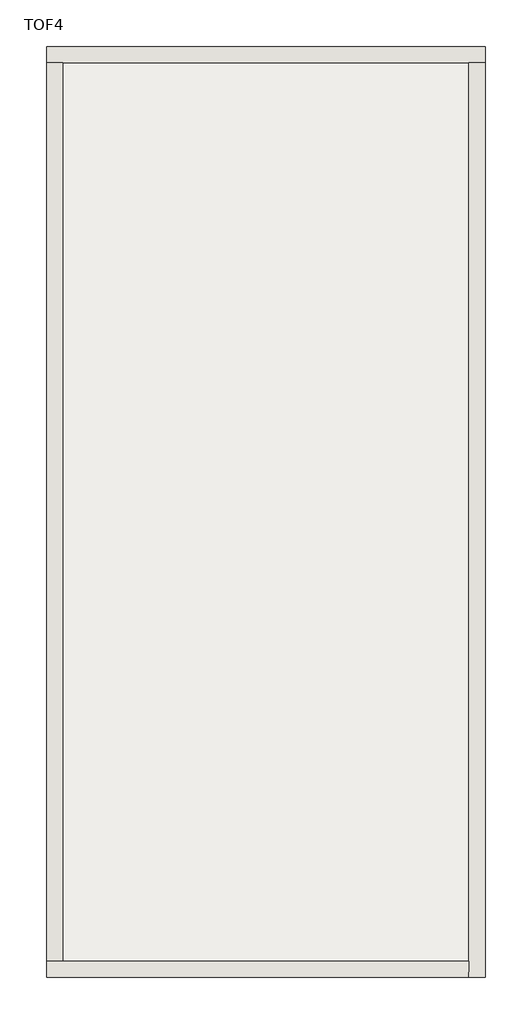
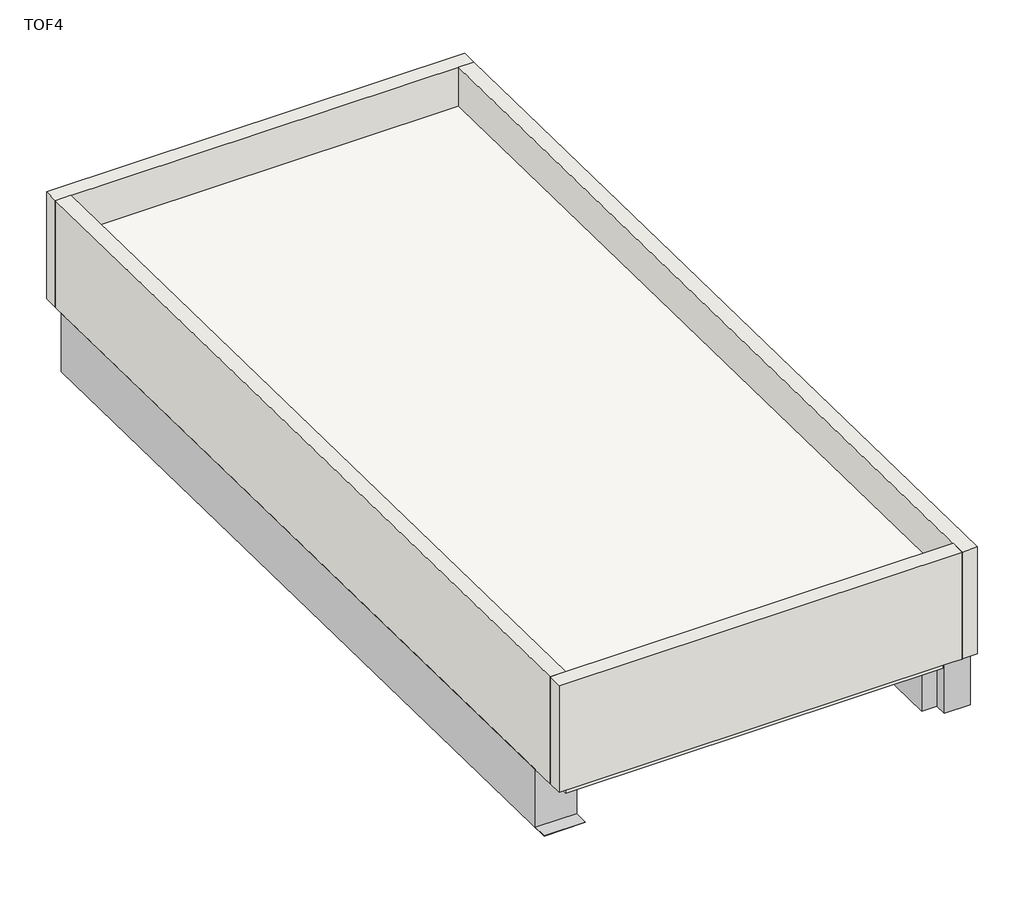
# One storey: 4 walls, 2 beams, 2 slabs.
"""IFC4 building model written with IfcOpenShell, lengths in millimetres."""

from ifc_helpers import new_model, si_unit, frame, origin, place, context, project, spatial, polyline, outline, extrude, faceted_brep, element, save

model = new_model("IFC4")

# Units and contexts
model_context = context("Model", 3, world=origin())
ifc_project = project(units=[si_unit("LENGTHUNIT", "METRE", prefix="MILLI")], contexts=[model_context])

# Site, building, storey
site = spatial("IfcSite", under=ifc_project)
building = spatial("IfcBuilding", under=site)
storey = spatial("IfcBuildingStorey", under=building, Name="TOF4", Elevation=19209.9618634)

# Beams
placement = place(None, origin())
element("IfcBeam", 1, ObjectType="RC Beam_Rectangular : H_SB_AR_S16_AG_B400xH600_PHWG1", at=placement, inside=storey, context=model_context, shape_type="Brep", body=[
    faceted_brep([(50825.0, 9549.5208589, 19206.0830755), (51225.0, 9549.5208589, 19206.0830755), (51225.0, 17599.5208589, 19049.9618634), (50825.0, 17599.5208589, 19049.9618634), (50825.0, 9549.5208589, 18609.9618634), (50825.0, 17549.5208589, 19049.9618634), (50825.0, 17549.5208589, 18450.8187335), (50825.0, 9399.5208589, 18608.8793395), (50825.0, 9399.5208589, 18609.9618634), (51225.0, 17549.5208589, 18450.8187335), (51225.0, 9399.5208589, 18608.8793395), (51225.0, 9549.5208589, 18609.9618634), (51225.0, 9399.5208589, 18609.9618634), (51225.0, 17549.5208589, 19049.9618634), (51075.0, 9549.5208589, 18609.9618634)], [[[0, 1, 2, 3]], [[4, 0, 3, 5, 6, 7, 8]], [[6, 9, 10, 7]], [[1, 11, 12, 10, 9, 13, 2]], [[11, 14, 4, 8, 12]], [[4, 14, 11, 1, 0]], [[5, 13, 9, 6]], [[13, 5, 3, 2]], [[8, 7, 10, 12]]]),
])
element("IfcBeam", 2, ObjectType="RC Beam_Rectangular : H_SB_AR_S16_AG_B400xH600_PHWG1", at=placement, inside=storey, context=model_context, shape_type="Brep", body=[
    faceted_brep([(54900.0, 9274.5208589, 19211.4164088), (54900.0, 17599.5208589, 19049.9618634), (54500.0, 17599.5208589, 19049.9618634), (54500.0, 9549.5208589, 19206.0830755), (54500.0, 9399.5208589, 19208.9921664), (54750.0, 9399.5208589, 19208.9921664), (54750.0, 9349.5208589, 19209.9618634), (54500.0, 9349.5208589, 19209.9618634), (54500.0, 9299.5208589, 19210.9315603), (54750.0, 9299.5208589, 19210.9315603), (54750.0, 9274.5208589, 19211.4164088), (54500.0, 9299.5208589, 19209.9618634), (54900.0, 17549.5208589, 18450.8187335), (54900.0, 9274.5208589, 18611.303582), (54650.0, 9274.5208589, 18611.303582), (54650.0, 9399.5208589, 18608.8793395), (54500.0, 9399.5208589, 18608.8793395), (54500.0, 17549.5208589, 18450.8187335), (54900.0, 17549.5208589, 19049.9618634), (54500.0, 17549.5208589, 19049.9618634), (54750.0, 9274.5208589, 19206.6647429), (54650.0, 9274.5208589, 19206.6647429), (54650.0, 9399.5208589, 19206.6647429), (54750.0, 9399.5208589, 19206.6647429), (54750.0, 9299.5208589, 19209.9618634)], [[[0, 1, 2, 3, 4, 5, 6, 7, 8, 9, 10]], [[8, 7, 11]], [[12, 13, 14, 15, 16, 17]], [[1, 0, 13, 12, 18]], [[19, 18, 12, 17]], [[18, 19, 2, 1]], [[13, 0, 10, 20, 21, 14]], [[22, 23, 5, 4, 16, 15]], [[7, 6, 24, 11]], [[23, 22, 21, 20]], [[22, 15, 14, 21]], [[5, 23, 20, 10, 9, 24, 6]], [[24, 9, 8, 11]], [[19, 17, 16, 4, 3, 2]]]),
])

# Slabs
element("IfcSlab", 3, ObjectType="H_FL_AR_S17_RC Slab T150_PHRS1", at=placement, inside=storey, context=model_context, shape_type="SweptSolid", body=[
    extrude(outline(polyline([(17649.5208589, 18899.9343282), (9299.5208589, 19059.9343282), (9299.5208589, 19209.9618634), (17649.5208589, 19049.9618634), (17649.5208589, 18899.9343282)])), frame((50975.0, 0.0, 0.0), z_axis=(1.0, 0.0, 0.0), x_axis=(0.0, 1.0, 0.0)), (0.0, 0.0, 1.0), 3775.0),
])
element("IfcSlab", 4, ObjectType="H_RF_AR_B06_Roof Finish", at=placement, inside=storey, context=model_context, shape_type="SweptSolid", body=[
    extrude(outline(polyline([(17649.5208589, 19399.8976154), (9299.4677289, 19559.8976154), (9299.4677289, 19909.9618634), (17649.5208589, 19749.9618634), (17649.5208589, 19399.8976154)])), frame((50975.0, 0.0, 0.0), z_axis=(1.0, 0.0, 0.0), x_axis=(0.0, 1.0, 0.0)), (0.0, 0.0, 1.0), 3775.0),
])

# Walls
element("IfcWall", 5, ObjectType="H_WA_AR_B02_Ext Wall_RC T150_parapet", at=placement, inside=storey, context=model_context, shape_type="SweptSolid", body=[
    extrude(outline(polyline([(19049.9618634, 51075.0), (19049.9618634, 54650.0), (19051.3766309, 54650.0), (19051.3766309, 54900.0), (20149.9618634, 54900.0), (20149.9618634, 50825.0), (19051.3766309, 50825.0), (19051.3766309, 51075.0), (19049.9618634, 51075.0)])), frame((0.0, 17649.5208589, 0.0), z_axis=(0.0, 1.0, 0.0), x_axis=(0.0, 0.0, 1.0)), (0.0, 0.0, 1.0), 150.0),
])
element("IfcWall", 6, ObjectType="H_WA_AR_B02_Ext Wall_RC T150_parapet", at=placement, inside=storey, context=model_context, shape_type="Brep", body=[
    faceted_brep([(54750.0, 17649.5208589, 20151.3736281), (54750.0, 17649.5208589, 19051.3736281), (54750.0, 9149.5208589, 19211.3736281), (54750.0, 9149.5208589, 20309.9618634), (54750.0, 9149.5208589, 20311.3736281), (54900.0, 17649.5208589, 19051.3736281), (54900.0, 17649.5208589, 20149.9618634), (54900.0, 17649.5208589, 20151.3736281), (54900.0, 9149.5208589, 20311.3736281), (54900.0, 9149.5208589, 19211.3736281), (54900.0, 17549.5208589, 19053.255981)], [[[0, 1, 2, 3, 4]], [[5, 6, 7, 8, 9, 10]], [[4, 3, 2, 9, 8]], [[2, 1, 5, 10, 9]], [[0, 4, 8, 7]], [[0, 7, 6, 5, 1]]]),
])
element("IfcWall", 7, ObjectType="H_WA_AR_B02_Ext Wall_RC T150_parapet", at=placement, inside=storey, context=model_context, shape_type="Brep", body=[
    faceted_brep([(54750.0, 9299.5208589, 19209.9618634), (54500.0, 9299.5208589, 19209.9618634), (50975.0, 9299.5208589, 19209.9618634), (50825.0, 9299.5208589, 19209.9618634), (50825.0, 9299.5208589, 20308.5500987), (50825.0, 9299.5208589, 20309.9618634), (54750.0, 9299.5208589, 20309.9618634), (54750.0, 9299.5208589, 19210.9315603), (54750.0, 9149.5208589, 19209.9618634), (54750.0, 9149.5208589, 19211.3736281), (54750.0, 9149.5208589, 20309.9618634), (50825.0, 9149.5208589, 20309.9618634), (50825.0, 9149.5208589, 19209.9618634), (50975.0, 9149.5208589, 19209.9618634), (54650.0, 9149.5208589, 19209.9618634)], [[[0, 1, 2, 3, 4, 5, 6, 7]], [[8, 9, 10, 11, 12, 13, 14]], [[3, 2, 1, 0, 8, 14, 13, 12]], [[6, 5, 11, 10]], [[0, 7, 6, 10, 9, 8]], [[5, 4, 3, 12, 11]]]),
])
element("IfcWall", 8, ObjectType="H_WA_AR_B02_Ext Wall_RC T150_parapet", at=placement, inside=storey, context=model_context, shape_type="Brep", body=[
    faceted_brep([(50975.0, 9299.5208589, 19208.5500987), (50975.0, 9399.5208589, 19206.6677457), (50975.0, 9549.5208589, 19203.8442163), (50975.0, 17649.5208589, 19051.3736281), (50975.0, 17649.5208589, 20151.3736281), (50975.0, 9299.5208589, 20308.5500987), (50975.0, 9299.5208589, 19209.9618634), (50825.0, 9299.5208589, 19208.5500987), (50825.0, 9299.5208589, 19209.9618634), (50825.0, 9299.5208589, 20308.5500987), (50825.0, 17649.5208589, 20151.3736281), (50825.0, 17649.5208589, 20149.9618634), (50825.0, 17649.5208589, 19051.3736281), (50825.0, 17549.5208589, 19053.255981), (50825.0, 9399.5208589, 19206.6677457)], [[[0, 1, 2, 3, 4, 5, 6]], [[7, 8, 9, 10, 11, 12, 13, 14]], [[0, 6, 5, 9, 8, 7]], [[3, 2, 1, 0, 7, 14, 13, 12]], [[5, 4, 10, 9]], [[3, 12, 11, 10, 4]]]),
])

save(model, "model.ifc")

# Revit data of these elements
# Type "RC Beam_Rectangular : H_SB_AR_S16_AG_B400xH600_PHWG1"
#   Type Comments = "CV-AG"
#   Type Mark = "PHWG1"
#   H_Q'ty Cal Type Tag = "SB-Q1"
#   H_WM Code_1 = "A03AF032-00022 |  | M3 | Concrete Work | Superstructure Work | Structural Concrete | Cement Type-1 | 25MPa ≤ F'c (Cylinder Strength) < 30MPa |  |  |  |  | A03AF032-00022 Concrete Work Superstructure Work Structural Concrete  Cement Type-1 25MPa ≤ F'c (Cylinder Strength) < 30MPa      |  F'c (Cylinder Strength) = 24MPa"
#   H_WM Code_2 = "A03AD037-00002 |  | TON | Concrete Work | Substructure Work | Rebar Work | Deformed Bar (Non-Coat.) | 400MPa<Fy≤470MPa |  |  |  |  | A03AD037-00002 Concrete Work Substructure Work Rebar Work Deformed Bar (Non-Coat.)  400MPa<Fy≤470MPa      | ASTM A615 GRADE 60 (Fy=420MPa)"
#   H_WM Code_3 = "A03AF036-00001 |  | M2 | Concrete Work | Superstructure Work | Form Work (1 time in use) | Flat Form | Dressed Lumber, Plywood or Steel Form(Wood Planks are not Allowed) incl. Chamfer |  |  |  | A03AF036-00001 Concrete Work Superstructure Work Form Work (1 time in use) Flat Form     Dressed Lumber, Plywood or Steel Form(Wood Planks are not Allowed) incl. Chamfer   |"
#   중앙부 하부근 = ""
#   중앙부 상부근 = ""
#   중앙부 보조근 = ""
#   중앙부 늑근 = ""
#   외단부 하부근 = ""
#   외단부 상부근 = ""
#   외단부 보조근 = ""
#   외단부 늑근 = ""
#   부호 = "TG2"
#   내단부 하부근 = ""
#   내단부 상부근 = ""
#   내단부 보조근 = ""
#   내단부 늑근 = ""
#   ALL 하부근 = "3-D20"
#   ALL 상부근 = "4-D20"
#   ALL 보조근 = ""
#   ALL 늑근 = "2-D10 @120"
#   H_Rebar ratio = 0.14
#   Width = 400 mm
#   Height = 600 mm
#   Length [instance default] = 1524 mm
#   b = 400 mm
#   h = 600 mm
#   hec_material3 [instance default] = none
#   hec_material2 [instance default] = none
#   hec_material1 [instance default] = none
#   Structural Material [instance default] = none
#   Assembly Code = ""
# Type "H_FL_AR_S17_RC Slab T150_PHRS1"
#   Keynote = ""
#   Type Comments = "CV-AG"
#   Description = ""
#   Type Mark = "PHRS1"
#   H_Q'ty Cal Type Tag = "FL-Q1"
#   H_WM Code_1 = "A03AF032-00025 |  | M3 | Concrete Work | Superstructure Work | Structural Concrete | Cement Type-1 | 20MPa ≤ F'c (Cylinder Strength) < 25MPa |  |  |  |  | A03AF032-00025 Concrete Work Superstructure Work Structural Concrete  Cement Type-1 20MPa ≤ F'c (Cylinder Strength) < 25MPa      |  F'c (Cylinder Strength) = 24MPa"
#   H_WM Code_2 = "A03AF037-00003 |  | TON | Concrete Work | Superstructure Work | Rebar Work | Deformed Bar (Non-Coat.) | 300MPa<Fy≤400MPa |  |  |  |  | A03AF037-00003 Concrete Work Superstructure Work Rebar Work Deformed Bar (Non-Coat.)  300MPa<Fy≤400MPa      | ASTM A615 GRADE 60 (Fy=420MPa)"
#   H_WM Code_3 = "A03AF036-00001 |  | M2 | Concrete Work | Superstructure Work | Form Work (1 time in use) | Flat Form | Dressed Lumber, Plywood or Steel Form(Wood Planks are not Allowed) incl. Chamfer |  |  |  | A03AF036-00001 Concrete Work Superstructure Work Form Work (1 time in use) Flat Form     Dressed Lumber, Plywood or Steel Form(Wood Planks are not Allowed) incl. Chamfer   |"
#   H_WM Code_4 = "A04AQ087-00002 |  | M2 | Finishing Work | Roof Work | Waterproofing Coating | Acrylic Polymer Protective Coating | only for Roof Area |  |  |  |  | A04AQ087-00002 Finishing Work Roof Work Waterproofing Coating Acrylic Polymer Protective Coating    only for Roof Area    | EPDM(or Equivalent)\nTHK=( 4 )mm"
#   H_WM Code_5 = "A04AQ088-00004 |  | M2 | Finishing Work | Roof Work | Roof Insulation | Rigid Extruded Polystyrene Foam Insulation |  | 100mm≤THK | THK=(  )mm |  | A04AQ088-00004 Finishing Work Roof Work Roof Insulation Rigid Extruded Polystyrene Foam Insulation       100mm≤THK | XPS\nTHK=( 220 )mm"
#   H_WM Code_6 = "A04AQ310-00001 |  | M2 | Finishing Work | Roof Work | Waterproofing Membrane | EPDM(or Equivalent) | w/ Accessories | THK=(  )mm |  | A04AQ310-00001 Finishing Work Roof Work Waterproofing Membrane EPDM(or Equivalent)     w/ Accessories   | Mesh Size=DIA( #8 )mm x ( 150 )mm x (150  )mm"
#   H_WM Code_7 = "A04AQ089-00001 |  | M3 | Finishing Work | Roof Work | Protective Concrete w/ Steel Trowel Finish |  |  |  | A04AQ089-00001 Finishing Work Roof Work Protective Concrete w/ Steel Trowel Finish         | Protective Concrete w/ Steel Trowel Finish"
#   H_Rebar ratio = 0.1
#   Function = 1
#   Layers, outside or top first: 150 mm "00_Concrete_Reinf. Conc." (function 1)
# Type "H_RF_AR_B06_Roof Finish"
#   Keynote = ""
#   Type Comments = ""
#   Description = ""
#   H_Q'ty Cal Type Tag = "WA-Q1"
#   H_WM Code_1 = "A03AF032-00022 |  | M3 | Concrete Work | Superstructure Work | Structural Concrete | Cement Type-1 | 25MPa ≤ F'c (Cylinder Strength) < 30MPa |  |  |  |  | A03AF032-00022 Concrete Work Superstructure Work Structural Concrete  Cement Type-1 25MPa ≤ F'c (Cylinder Strength) < 30MPa      |"
#   H_WM Code_2 = "A03AD037-00002 |  | TON | Concrete Work | Substructure Work | Rebar Work | Deformed Bar (Non-Coat.) | 400MPa<Fy≤470MPa |  |  |  |  | A03AD037-00002 Concrete Work Substructure Work Rebar Work Deformed Bar (Non-Coat.)  400MPa<Fy≤470MPa      |"
#   H_WM Code_3 = "A03AD035-00001 |  | M2 | Concrete Work | Substructure Work | Form Work (3 times in use) | Flat Form | Dressed Lumber, Plywood or Steel Form(Wood Planks are not Allowed) incl. Chamfer |  |  |  | A03AD035-00001 Concrete Work Substructure Work Form Work (3 times in use) Flat Form     Dressed Lumber, Plywood or Steel Form(Wood Planks are not Allowed) incl. Chamfer   |"
#   H_WM Code_4 = "A03AH056-00001 |  | M2 | Concrete Work | Concrete Protective Coating (U/G) | Bitumen/Bituminous/Asphalt Coating |  |  | A03AH056-00001 Concrete Work Concrete Protective Coating (U/G) Bitumen/Bituminous/Asphalt Coating         | Exterior Protection"
#   H_WM Code_5 = "A03AD047-00004 |  | M2 | Concrete Work | Substructure Work | Insulation under Ground Floor | Extruded Polystyrene Insulation Board |  | 100mm≤THK | THK=(  )mm |  | A03AD047-00004 Concrete Work Substructure Work Insulation under Ground Floor Extruded Polystyrene Insulation Board       100mm≤THK | Interior Paint"
#   Function = 1
#   Layers, outside or top first: 350 mm "Roofs" (function 4)
# Type "H_WA_AR_B02_Ext Wall_RC T150_parapet"
#   Type Comments = "CV-AG"
#   Type Mark = "parapet"
#   H_Q'ty Cal Type Tag = "WA-Q1"
#   H_WM Code_1 = "A04AS178-00001 |  | M2 | Finishing Work | Exterior/Interior Finish Work | Gypsumboard Partition Wall (Removable Type) | Fire Protective Rating: N/A, 1-Layer Gypsum Board to Both Sides | Mineral Wool (Rock Wool) | Including Supporting Frame(Stud) & Accessories | 1-Layer Gypsumboard THK=9.5mm | Insulation THK=(  )mm |  | A04AS178-00001 Finishing Work Exterior/Interior Finish Work Gypsumboard Partition Wall (Removable Type) Fire Protective Rating: N/A, 1-Layer Gypsum Board to Both Sides   Mineral Wool (Rock Wool)  Including Supporting Frame(Stud) & Accessories  1-Layer Gypsumboard THK=9.5mm | Glass wall (WM 없음)"
#   H_WM Code_2 = "A03AD037-00002 |  | TON | Concrete Work | Substructure Work | Rebar Work | Deformed Bar (Non-Coat.) | 400MPa<Fy≤470MPa |  |  |  |  | A03AD037-00002 Concrete Work Substructure Work Rebar Work Deformed Bar (Non-Coat.)  400MPa<Fy≤470MPa      | ASTM A615 GRADE 60 (Fy=420MPa)"
#   H_WM Code_3 = "A03AD035-00001 |  | M2 | Concrete Work | Substructure Work | Form Work (3 times in use) | Flat Form | Dressed Lumber, Plywood or Steel Form(Wood Planks are not Allowed) incl. Chamfer |  |  |  | A03AD035-00001 Concrete Work Substructure Work Form Work (3 times in use) Flat Form     Dressed Lumber, Plywood or Steel Form(Wood Planks are not Allowed) incl. Chamfer   |"
#   H_WM Code_4 = "A03AH056-00001 |  | M2 | Concrete Work | Concrete Protective Coating (U/G) | Bitumen/Bituminous/Asphalt Coating |  |  | A03AH056-00001 Concrete Work Concrete Protective Coating (U/G) Bitumen/Bituminous/Asphalt Coating         |"
#   H_WM Code_5 = "A01ZZ003-00001 |  | M3 | Earth Work | - | Backfill | Re-use, Soil |  |  |  | Compaction=(  )% |  | A01ZZ003-00001 Earth Work - Backfill Re-use, Soil        | Compaction=( 95 )%"
#   H_WM Code_6 = "A01ZZ004-00001 |  | M3 | Earth Work | - | Disposal | Soil |  |  |  | Disposal Distance=Appx. (  )km from Site |  | A01ZZ004-00001 Earth Work - Disposal Soil        | Disposal Distance=Appx. (20 )km from Site"
#   H_Rebar ratio = 0.12
#   Layers, outside or top first: 150 mm "00_Concrete_Reinf. Conc." (function 1)
# Elements 1, 2 (IfcBeam, "RC Beam_Rectangular : H_SB_AR_S16_AG_B400xH600_PHWG1")
#   Comments = ""
#   hec_material3 = none
#   hec_material2 = none
#   hec_material1 = none
#   Structural Material = 00_Concrete_Reinf. Conc.
#   Phase Created = New Construction
#   Materials on its faces: "00_Concrete_Reinf. Conc."
# Element 3 (IfcSlab, "H_FL_AR_S17_RC Slab T150_PHRS1")
#   Comments = ""
#   TMP_Element Name = "SS2"
#   Height Offset From Level = 0 mm
#   built-in parameter 1001954 = 1
#   Phase Created = New Construction
#   Materials on its faces: "00_Concrete_Reinf. Conc."
# Element 4 (IfcSlab, "H_RF_AR_B06_Roof Finish")
#   Height Offset From Level = 350 mm
#   Phase Created = New Construction
#   Materials on its faces: "Roofs"
# Element 5 (IfcWall, "H_WA_AR_B02_Ext Wall_RC T150_parapet")
#   Comments = ""
#   built-in parameter 1001111 = -160 mm
#   Top Offset = 150 mm
#   Base Offset = -160 mm
#   Unconnected Height = 1100 mm
#   wall height = 1100 mm
#   Phase Created = New Construction
#   Base Constraint = TOF4
#   Materials on its faces: "00_Concrete_Reinf. Conc."
# Elements 6, 7, 8 (IfcWall, "H_WA_AR_B02_Ext Wall_RC T150_parapet")
#   Comments = ""
#   Top Offset = 150 mm
#   Base Offset = 0 mm
#   Unconnected Height = 1100 mm
#   wall height = 1100 mm
#   Phase Created = New Construction
#   Base Constraint = TOF4
#   Materials on its faces: "00_Concrete_Reinf. Conc."
# Materials
#   "00_Concrete_Reinf. Conc.": class "Concrete", colour RGB 176 176 176, transparency 0, Description = "Reinf. Conc.", Cost = 0, Image = Concrete.Cast-In-Place.Flat.Polished.Grey.jpg
#   "Roofs": class "Unassigned", colour RGB 38 15 153, transparency 0.5
